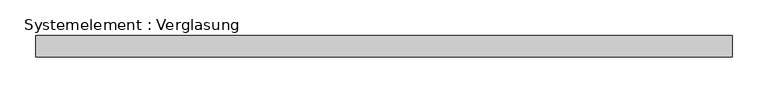
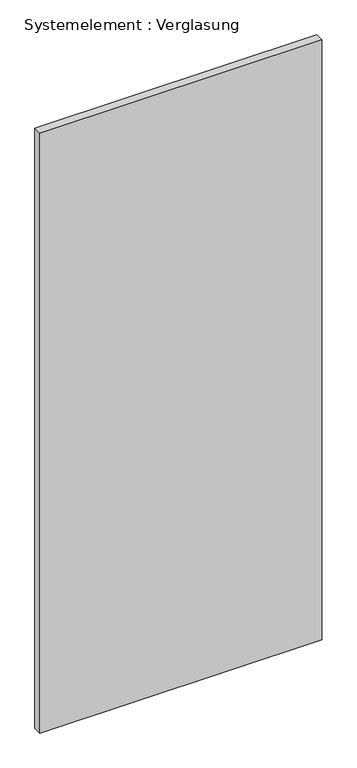
"""IFC4 building model written with IfcOpenShell, lengths in millimetres: plate geometry, Systemelement : Verglasung."""

import ifcopenshell
import ifcopenshell.guid

model = None  # the IFC model being written
_history = None  # IfcOwnerHistory: only IFC2X3 demands one
_inside = {}  # id of a spatial element -> (the spatial element, [elements in it])
_under = {}  # id of a project, library or spatial element -> (it, [spatial elements below it])
_declared = {}  # id of a project -> (the project, [libraries it declares])
_typed = {}  # id of a type object -> (the type object, [elements of that type])
_made_of = {}  # id of a material, layer set ... -> (it, [elements and type objects made of it])


def new_model(schema):
    """Start an empty IFC model of exactly this schema.

    Asked for "IFC4X3", IfcOpenShell would pick the latest addendum, in which some entities
    have other attributes; the version numbers below select the first issue.
    IFC2X3 requires an IfcOwnerHistory on every rooted entity: one is made here for all.
    """
    global model, _history
    if schema == "IFC4X3":
        model = ifcopenshell.file(schema_version=(4, 3, 0, 0))
    else:
        model = ifcopenshell.file(schema=schema)
    _inside.clear()
    _under.clear()
    _declared.clear()
    _typed.clear()
    _made_of.clear()
    _history = None
    if model.schema == "IFC2X3":
        org = make("IfcOrganization", Name="unknown")
        user = make(
            "IfcPersonAndOrganization",
            ThePerson=make("IfcPerson", FamilyName="unknown"),
            TheOrganization=org,
        )
        app = make(
            "IfcApplication",
            ApplicationDeveloper=org,
            Version="unknown",
            ApplicationFullName="unknown",
            ApplicationIdentifier="unknown",
        )
        _history = make(
            "IfcOwnerHistory",
            OwningUser=user,
            OwningApplication=app,
            ChangeAction="ADDED",
            CreationDate=0,
        )
    return model


def make(cls, **values):
    """One entity of the class cls with the attributes given. An attribute that is None is left unset."""
    return model.create_entity(
        cls, **{name: value for name, value in values.items() if value is not None}
    )


def rooted(cls, **values):
    """An entity with a GlobalId (a new one), such as an element, a storey or a relation."""
    return make(cls, GlobalId=ifcopenshell.guid.new(), OwnerHistory=_history, **values)


def si_unit(unit_type, name, prefix=None):
    """IfcSIUnit, for example si_unit("LENGTHUNIT", "METRE", prefix="MILLI")."""
    return make("IfcSIUnit", UnitType=unit_type, Prefix=prefix, Name=name)


def assignment(units):
    """IfcUnitAssignment: the units of a project."""
    return None if units is None else make("IfcUnitAssignment", Units=units)


def point(xyz):
    """IfcCartesianPoint."""
    return None if xyz is None else make("IfcCartesianPoint", Coordinates=xyz)


def direction(xyz):
    """IfcDirection."""
    return None if xyz is None else make("IfcDirection", DirectionRatios=xyz)


def frame(location, z_axis=None, x_axis=None):
    """IfcAxis2Placement3D, a coordinate frame: its origin and axes. An axis left out is left unset."""
    return make(
        "IfcAxis2Placement3D",
        Location=point(location),
        Axis=direction(z_axis),
        RefDirection=direction(x_axis),
    )


def origin():
    """The frame at (0, 0, 0) with its axes left unset."""
    return frame((0.0, 0.0, 0.0))


def origin_with_axes():
    """The frame at (0, 0, 0) with the z axis (0, 0, 1) and the x axis (1, 0, 0) written out."""
    return frame((0.0, 0.0, 0.0), z_axis=(0.0, 0.0, 1.0), x_axis=(1.0, 0.0, 0.0))


def place(relative_to, where):
    """IfcLocalPlacement: puts the frame where relative to a parent placement (None: the world)."""
    return make(
        "IfcLocalPlacement", PlacementRelTo=relative_to, RelativePlacement=where
    )


def context(
    kind, dimensions, precision=None, world=None, true_north=None, identifier=None
):
    """IfcGeometricRepresentationContext, for example the 3D "Model" context."""
    return make(
        "IfcGeometricRepresentationContext",
        ContextIdentifier=identifier,
        ContextType=kind,
        CoordinateSpaceDimension=dimensions,
        Precision=precision,
        WorldCoordinateSystem=world,
        TrueNorth=true_north,
    )


def project(units=None, contexts=None):
    """IfcProject with its units and contexts."""
    return rooted(
        "IfcProject",
        Name="project",
        RepresentationContexts=contexts,
        UnitsInContext=assignment(units),
    )


def spatial(cls, under=None, at=None, **own):
    """A site, building, storey or space (cls), placed at a placement, below another one or the project."""
    s = rooted(cls, ObjectPlacement=at, **own)
    if under is not None:
        _under.setdefault(under.id(), (under, []))[1].append(s)
    return s


def polyline(points):
    """IfcPolyline through the points."""
    return make("IfcPolyline", Points=[point(p) for p in points])


def outline(outer, holes=None, kind="AREA"):
    """IfcArbitraryClosedProfileDef: a profile drawn as a closed curve; with holes, ...WithVoids."""
    if holes is None:
        return make("IfcArbitraryClosedProfileDef", ProfileType=kind, OuterCurve=outer)
    return make(
        "IfcArbitraryProfileDefWithVoids",
        ProfileType=kind,
        OuterCurve=outer,
        InnerCurves=holes,
    )


def extrude(swept, where, along, depth):
    """IfcExtrudedAreaSolid: the profile swept, set in the frame where, extruded along a direction by depth."""
    return make(
        "IfcExtrudedAreaSolid",
        SweptArea=swept,
        Position=where,
        ExtrudedDirection=direction(along),
        Depth=depth,
    )


def shape(context_of_items, identifier, shape_type, items):
    """IfcShapeRepresentation: the items that make up one representation, for example the "Body"."""
    return make(
        "IfcShapeRepresentation",
        ContextOfItems=context_of_items,
        RepresentationIdentifier=identifier,
        RepresentationType=shape_type,
        Items=items,
    )


def source(mapping_origin, context_of_items, identifier, shape_type, items):
    """IfcRepresentationMap: a shape defined once, which mapped items show again and again."""
    return make(
        "IfcRepresentationMap",
        MappingOrigin=mapping_origin,
        MappedRepresentation=shape(context_of_items, identifier, shape_type, items),
    )


def transform(
    local_origin,
    x_axis=None,
    y_axis=None,
    z_axis=None,
    scale=None,
    scale2=None,
    scale3=None,
    uniform=True,
):
    """IfcCartesianTransformationOperator3D, or its non-uniform kind. x_axis, y_axis, z_axis: its Axis1, 2, 3."""
    if uniform:
        return make(
            "IfcCartesianTransformationOperator3D",
            Axis1=direction(x_axis),
            Axis2=direction(y_axis),
            LocalOrigin=point(local_origin),
            Scale=scale,
            Axis3=direction(z_axis),
        )
    return make(
        "IfcCartesianTransformationOperator3DnonUniform",
        Axis1=direction(x_axis),
        Axis2=direction(y_axis),
        LocalOrigin=point(local_origin),
        Scale=scale,
        Axis3=direction(z_axis),
        Scale2=scale2,
        Scale3=scale3,
    )


def mapped(mapping_source, mapping_target):
    """IfcMappedItem: shows the shape of a source again, moved by a transform."""
    return make(
        "IfcMappedItem", MappingSource=mapping_source, MappingTarget=mapping_target
    )


def made_of(thing, what):
    """Note that an element or type object is made of a material, layer set ...; save() writes the relation."""
    if what is not None:
        _made_of.setdefault(what.id(), (what, []))[1].append(thing)
    return thing


def element(
    cls,
    number,
    at=None,
    inside=None,
    cuts=None,
    type_object=None,
    material=None,
    context=None,
    identifier="Body",
    shape_type=None,
    held_by="IfcProductDefinitionShape",
    body=None,
    shapes=None,
    **own,
):
    """One element of the class cls, such as IfcWall. Its Tag is "e" and its number.

    at: its placement. inside: the storey or other place that contains it. cuts: it is an
    opening in that element (IfcRelVoidsElement). A single representation is given by context,
    identifier, shape_type and body (its items); several are given by shapes. held_by: the class
    of the entity that holds the representations. save() writes the other relations.
    """
    e = rooted(cls, Tag="e%d" % number, ObjectPlacement=at, **own)
    if body is not None:
        shapes = [shape(context, identifier, shape_type, body)]
    if shapes is not None:
        e.Representation = make(held_by, Representations=shapes)
    if inside is not None:
        _inside.setdefault(inside.id(), (inside, []))[1].append(e)
    if cuts is not None:
        rooted(
            "IfcRelVoidsElement", RelatingBuildingElement=cuts, RelatedOpeningElement=e
        )
    if type_object is not None:
        _typed.setdefault(type_object.id(), (type_object, []))[1].append(e)
    return made_of(e, material)


def aggregate(whole, parts):
    """IfcRelAggregates: a whole, such as a stair, and the parts it consists of."""
    return rooted("IfcRelAggregates", RelatingObject=whole, RelatedObjects=parts)


def save(model, path):
    """Write the relations noted so far, then the file.

    IfcRelAggregates (storeys below a building ...), IfcRelContainedInSpatialStructure (elements
    in a storey), IfcRelDefinesByType, IfcRelAssociatesMaterial and IfcRelDeclares: one each for
    every whole, place, type object, material and project.
    """
    for whole, parts in _under.values():
        aggregate(whole, parts)
    for where, things in _inside.values():
        rooted(
            "IfcRelContainedInSpatialStructure",
            RelatedElements=things,
            RelatingStructure=where,
        )
    for kind, things in _typed.values():
        rooted("IfcRelDefinesByType", RelatedObjects=things, RelatingType=kind)
    for what, things in _made_of.values():
        rooted("IfcRelAssociatesMaterial", RelatedObjects=things, RelatingMaterial=what)
    for by, libraries in _declared.values():
        rooted("IfcRelDeclares", RelatingContext=by, RelatedDefinitions=libraries)
    model.write(path)


def systemelement_verglasung_a6efefe2(model_context):
    return source(origin(), model_context, "Body", "SweptSolid", [
        extrude(outline(polyline([(486.6118989, -15.0), (-486.6118989, -15.0), (-486.6118989, 15.0), (486.6118989, 15.0), (486.6118989, -15.0)])), origin_with_axes(), (0.0, 0.0, 1.0), 2190.0),
    ])


if __name__ == "__main__":
    model = new_model("IFC4")
    model_context = context("Model", 3, world=origin())
    ifc_project = project(units=[si_unit("LENGTHUNIT", "METRE", prefix="MILLI")], contexts=[model_context])
    site = spatial("IfcSite", under=ifc_project)
    building = spatial("IfcBuilding", under=site)
    placement = place(None, origin())
    systemelement_verglasung_shape = systemelement_verglasung_a6efefe2(model_context)
    element("IfcPlate", 1, ObjectType="Systemelement : Verglasung", at=placement, inside=building, context=model_context, shape_type="MappedRepresentation", body=[
        mapped(systemelement_verglasung_shape, transform((0.0, 0.0, 0.0), x_axis=(1.0, 0.0, 0.0), y_axis=(0.0, 1.0, 0.0), z_axis=(0.0, 0.0, 1.0))),
    ])
    save(model, "model.ifc")

# Revit data of these elements
# Type "Systemelement : Verglasung"
#   Construction Type Id = "GSP4R"
#   Analytic Construction = "1/8 Zoll Pilkington-Verglasung einfach"
#   Visual Light Transmittance = 0.9
#   Solar Heat Gain Coefficient = 0.86
#   Heat Transfer Coefficient (U) = 6.7069 W/(m²·K)
# Element 1 (IfcPlate, "Systemelement : Verglasung")
#   Materials on its faces: "Glas"
# Materials
#   "Glas": class "Glas", colour RGB 0 0 255, transparency 0.75, Comments = "Render-Darstellung nicht aktualisiert ", Cost = 0
